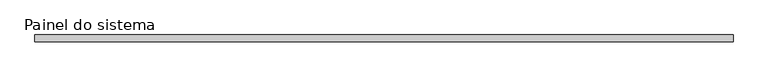
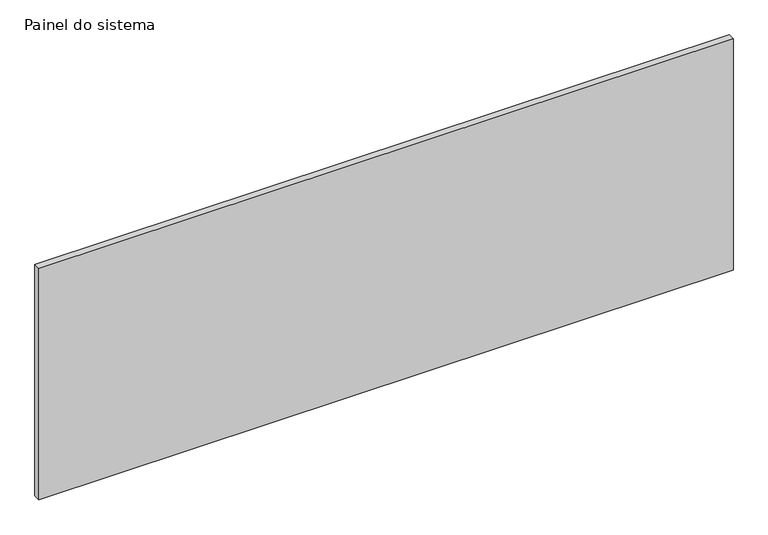
"""IFC4 building model written with IfcOpenShell, lengths in millimetres: plate geometry, Painel do sistema : Envidraçado."""

from ifc_helpers import new_model, si_unit, origin, origin_with_axes, place, context, project, spatial, polyline, outline, extrude, source, transform, mapped, element, save


def painel_do_sistema_e2dfd561(model_context):
    return source(origin(), model_context, "Body", "SweptSolid", [
        extrude(outline(polyline([(1275.8375317, -49.5), (-1275.8375317, -49.5), (-1275.8375317, -24.5), (1275.8375317, -24.5), (1275.8375317, -49.5)])), origin_with_axes(), (0.0, 0.0, 1.0), 900.0),
    ])


if __name__ == "__main__":
    model = new_model("IFC4")
    model_context = context("Model", 3, world=origin())
    ifc_project = project(units=[si_unit("LENGTHUNIT", "METRE", prefix="MILLI")], contexts=[model_context])
    site = spatial("IfcSite", under=ifc_project)
    building = spatial("IfcBuilding", under=site)
    placement = place(None, origin())
    painel_do_sistema_shape = painel_do_sistema_e2dfd561(model_context)
    element("IfcPlate", 1, ObjectType="Painel do sistema : Envidraçado", at=placement, inside=building, context=model_context, shape_type="MappedRepresentation", body=[
        mapped(painel_do_sistema_shape, transform((0.0, 0.0, 0.0), x_axis=(1.0, 0.0, 0.0), y_axis=(0.0, 1.0, 0.0), z_axis=(0.0, 0.0, 1.0))),
    ])
    save(model, "model.ifc")

# Revit data of these elements
# Type "Painel do sistema : Envidraçado"
#   Construction Type Id = "GSP4R"
#   Analytic Construction = "Vidraça única Pilkington 1/8 pol"
#   Visual Light Transmittance = 0.9
#   Solar Heat Gain Coefficient = 0.86
#   Heat Transfer Coefficient (U) = 6.7069 W/(m²·K)
# Element 1 (IfcPlate, "Painel do sistema : Envidraçado")
#   Materials on its faces: "Vidro"
# Materials
#   "Vidro": class "Vidro", colour RGB 0 128 192, transparency 0.9, Description = "Vidro de sílica", Cost = 0
